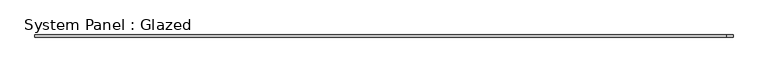
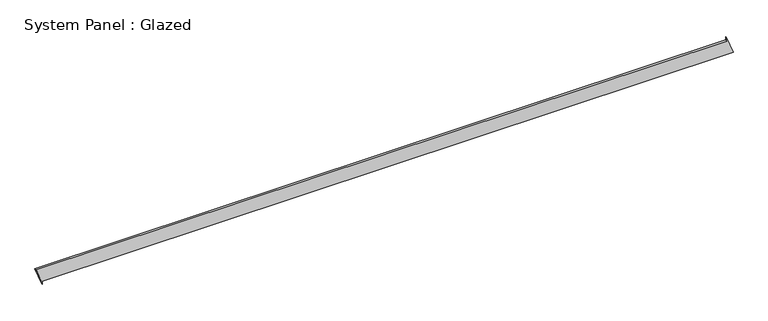
"""IFC4 building model written with IfcOpenShell, lengths in millimetres: plate geometry, System Panel : Glazed."""

from ifc_helpers import new_model, si_unit, frame, origin, place, context, project, spatial, polyline, outline, extrude, source, transform, mapped, element, save


def system_panel_glazed_7ff1da7a(model_context):
    return source(origin(), model_context, "Body", "SweptSolid", [
        extrude(outline(polyline([(0.0, -3956.991033), (35.3553391, -3956.991033), (35.3553391, 4027.528574), (233.766037, 3956.5208191), (198.410698, 3956.5199259), (198.6124026, -4027.528574), (0.0, -3956.991033)])), frame((0.0, -49.5, 0.0), z_axis=(0.0, 1.0, 0.0), x_axis=(0.0, 0.0, 1.0)), (0.0, 0.0, 1.0), 25.0),
    ])


if __name__ == "__main__":
    model = new_model("IFC4")
    model_context = context("Model", 3, world=origin())
    ifc_project = project(units=[si_unit("LENGTHUNIT", "METRE", prefix="MILLI")], contexts=[model_context])
    site = spatial("IfcSite", under=ifc_project)
    building = spatial("IfcBuilding", under=site)
    placement = place(None, origin())
    system_panel_glazed_shape = system_panel_glazed_7ff1da7a(model_context)
    element("IfcPlate", 1, ObjectType="System Panel : Glazed", at=placement, inside=building, context=model_context, shape_type="MappedRepresentation", body=[
        mapped(system_panel_glazed_shape, transform((0.0, 0.0, 0.0), x_axis=(1.0, 0.0, 0.0), y_axis=(0.0, 1.0, 0.0), z_axis=(0.0, 0.0, 1.0))),
    ])
    save(model, "model.ifc")

# Revit data of these elements
# Element 1 (IfcPlate, "System Panel : Glazed")
#   Materials on its faces: "Glass"
# Materials
#   "Glass": class "Glass", colour RGB 218 227 224, transparency 0.85, Description = "Soda Lime Glass", Cost = 0
